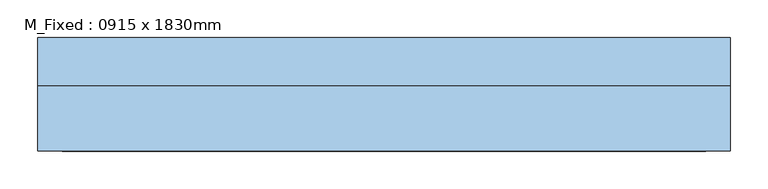
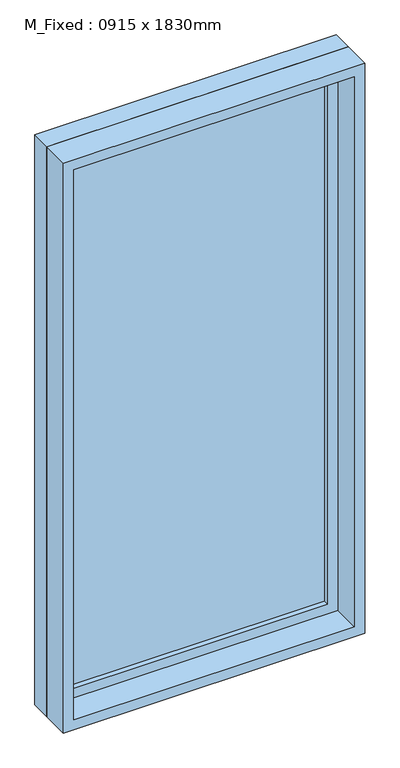
"""IFC4 building model written with IfcOpenShell, lengths in millimetres: window geometry, M_Fixed : 0915 x 1830mm."""

from ifc_helpers import new_model, si_unit, frame, origin, place, context, project, spatial, polyline, outline, extrude, source, transform, mapped, element, save


def m_fixed_0915_x_1830mm_81dddaff(model_context):
    return source(origin(), model_context, "Body", "SweptSolid", [
        extrude(outline(polyline([(-394.5, 53.0), (394.5, 53.0), (394.5, 41.0), (-394.5, 41.0), (-394.5, 53.0)])), frame((0.0, 0.0, 368.0), z_axis=(0.0, 0.0, 1.0), x_axis=(1.0, 0.0, 0.0)), (0.0, 0.0, 1.0), 1704.0),
        extrude(outline(polyline([(2116.0, -438.5), (324.0, -438.5), (324.0, 438.5), (2116.0, 438.5), (2116.0, -438.5)]), holes=[polyline([(2072.0, -394.5), (2072.0, 394.5), (368.0, 394.5), (368.0, -394.5), (2072.0, -394.5)])]), frame((0.0, 25.0, 0.0), z_axis=(0.0, 1.0, 0.0), x_axis=(0.0, 0.0, 1.0)), (0.0, 0.0, 1.0), 44.0),
        extrude(outline(polyline([(2135.0, -457.5), (305.0, -457.5), (305.0, 457.5), (2135.0, 457.5), (2135.0, -457.5)]), holes=[polyline([(2116.0, -438.5), (2116.0, 438.5), (324.0, 438.5), (324.0, -438.5), (2116.0, -438.5)])]), frame((0.0, 25.0, 0.0), z_axis=(0.0, 1.0, 0.0), x_axis=(0.0, 0.0, 1.0)), (0.0, 0.0, 1.0), 63.0),
        extrude(outline(polyline([(2135.0, -457.5), (305.0, -457.5), (305.0, 457.5), (2135.0, 457.5), (2135.0, -457.5)]), holes=[polyline([(2103.0, -425.5), (2103.0, 425.5), (337.0, 425.5), (337.0, -425.5), (2103.0, -425.5)])]), frame((0.0, -62.0, 0.0), z_axis=(0.0, 1.0, 0.0), x_axis=(0.0, 0.0, 1.0)), (0.0, 0.0, 1.0), 87.0),
    ])


if __name__ == "__main__":
    model = new_model("IFC4")
    model_context = context("Model", 3, world=origin())
    ifc_project = project(units=[si_unit("LENGTHUNIT", "METRE", prefix="MILLI")], contexts=[model_context])
    site = spatial("IfcSite", under=ifc_project)
    building = spatial("IfcBuilding", under=site)
    placement = place(None, origin())
    m_fixed_0915_x_1830mm_shape = m_fixed_0915_x_1830mm_81dddaff(model_context)
    element("IfcWindow", 1, ObjectType="M_Fixed : 0915 x 1830mm", at=placement, inside=building, context=model_context, shape_type="MappedRepresentation", body=[
        mapped(m_fixed_0915_x_1830mm_shape, transform((0.0, 0.0, 0.0), x_axis=(1.0, 0.0, 0.0), y_axis=(0.0, 1.0, 0.0), z_axis=(0.0, 0.0, 1.0))),
    ])
    save(model, "model.ifc")

# Revit data of these elements
# Type "M_Fixed : 0915 x 1830mm"
#   Type Mark = "18"
#   Height = 1.83 m
#   Default Sill Height = 0.305 m
#   Width = 0.915 m
#   Window Inset = 0.019 m
#   Frame Exterior Material = Sash
#   Frame Interior Material = Sash
#   Glass Pane Material = Glass
#   Sash = Sash
#   Wall Closure = (empty or 0)
# Element 1 (IfcWindow, "M_Fixed : 0915 x 1830mm")
#   Materials on its faces: "Sash", "Glass"
# Materials
#   "Sash": class "Wood", colour RGB 136 99 55, transparency 0
#   "Glass": class "Glass", colour RGB 247 249 248, transparency 0.85, Description = "Soda Lime Glass", Cost = 0
